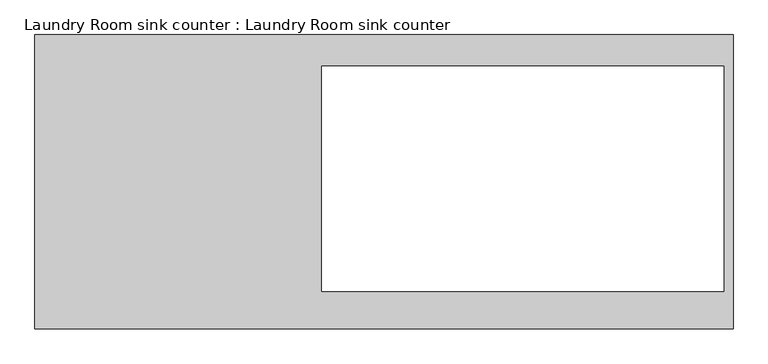
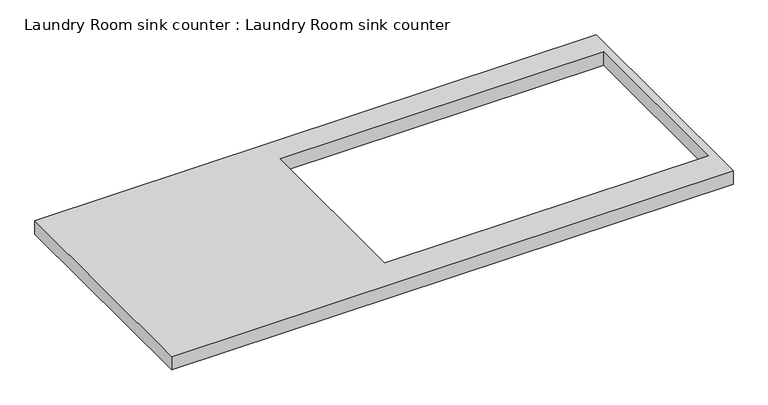
"""IFC4 building model written with IfcOpenShell, lengths in millimetres: furniture geometry, Laundry Room sink counter : Laundry Room sink counter."""

from ifc_helpers import new_model, si_unit, frame, origin, place, context, project, spatial, polyline, outline, extrude, source, transform, mapped, element, save


def laundry_room_sink_counter_laundry_room_sink_counter_54500054(model_context):
    return source(origin(), model_context, "Body", "SweptSolid", [
        extrude(outline(polyline([(10633.032173, 11758.3915372), (12150.1020554, 11758.3915372), (12150.1020554, 11118.9465372), (10633.032173, 11118.9465372), (10633.032173, 11758.3915372)]), holes=[polyline([(12130.0299078, 11690.1441273), (11256.6350363, 11690.1441273), (11256.6350363, 11200.7027872), (12130.0299078, 11200.7027872), (12130.0299078, 11690.1441273)])]), frame((0.0, 0.0, 876.3), z_axis=(0.0, 0.0, 1.0), x_axis=(1.0, 0.0, 0.0)), (0.0, 0.0, 1.0), 38.1),
    ])


if __name__ == "__main__":
    model = new_model("IFC4")
    model_context = context("Model", 3, world=origin())
    ifc_project = project(units=[si_unit("LENGTHUNIT", "METRE", prefix="MILLI")], contexts=[model_context])
    site = spatial("IfcSite", under=ifc_project)
    building = spatial("IfcBuilding", under=site)
    placement = place(None, origin())
    laundry_room_sink_counter_laundry_room_sink_counter_shape = laundry_room_sink_counter_laundry_room_sink_counter_54500054(model_context)
    element("IfcFurniture", 1, ObjectType="Laundry Room sink counter : Laundry Room sink counter", at=placement, inside=building, context=model_context, shape_type="MappedRepresentation", body=[
        mapped(laundry_room_sink_counter_laundry_room_sink_counter_shape, transform((0.0, 0.0, 0.0), x_axis=(1.0, 0.0, 0.0), y_axis=(0.0, 1.0, 0.0), z_axis=(0.0, 0.0, 1.0))),
    ])
    save(model, "model.ifc")

# Revit data of these elements
# Type "Laundry Room sink counter : Laundry Room sink counter"
#   COBie.Type = no
# Element 1 (IfcFurniture, "Laundry Room sink counter : Laundry Room sink counter")
#   Materials on its faces: "Corian - Dusk"
# Materials
#   "Corian - Dusk": class "Plastic", colour RGB 75 95 146, transparency 0, Manufacturer = "Corning", Cost = 0
